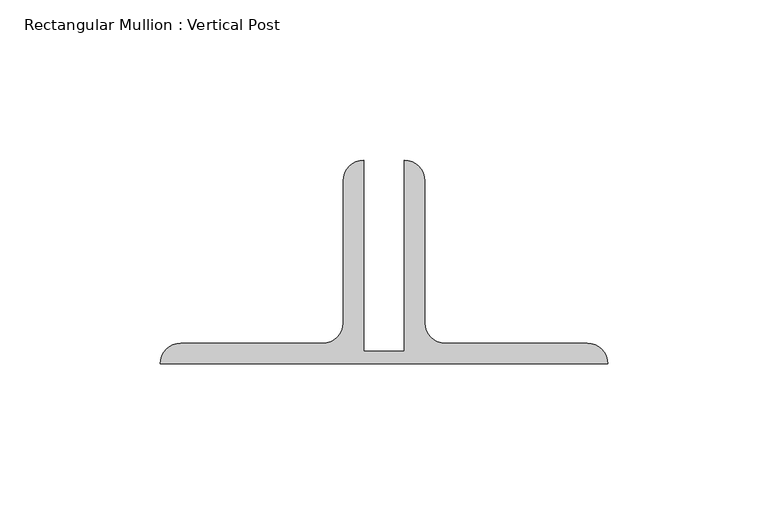
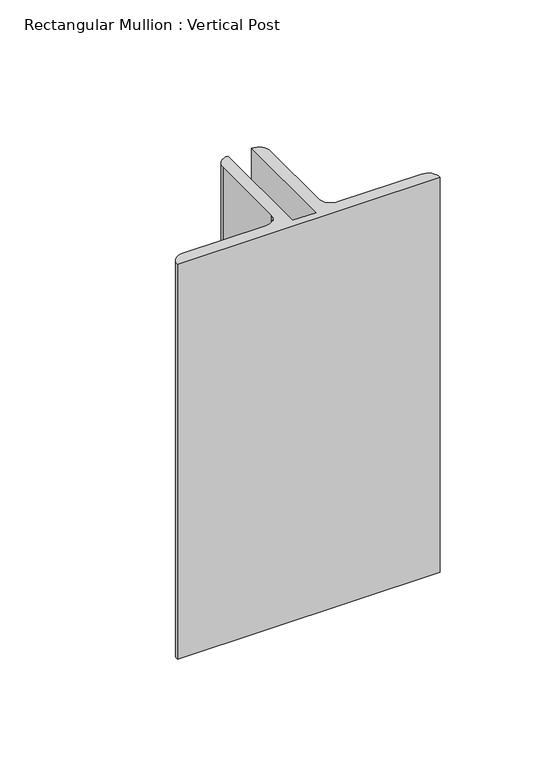
"""IFC4 building model written with IfcOpenShell, lengths in millimetres: member geometry, Rectangular Mullion : Vertical Post."""

from ifc_helpers import new_model, si_unit, point, frame, frame_2d, origin, place, context, project, spatial, polyline, circle_curve, trimmed, segment, composite_curve, outline, extrude, source, transform, mapped, element, save


def rectangular_mullion_vertical_post_21cc10da(model_context):
    return source(origin(), model_context, "Body", "SweptSolid", [
        extrude(outline(composite_curve([segment(polyline([(-76.2, 22.9145205), (-63.5, 22.9145205), (-63.5, 82.55)]), True, "CONTINUOUS"), segment(trimmed(circle_curve(frame_2d((-63.5, 76.2)), 6.35), [point((-63.5, 82.55))], [point((-57.15, 76.2))], False, "CARTESIAN"), True, "CONTINUOUS"), segment(polyline([(-57.15, 76.2), (-57.15, 31.75)]), True, "CONTINUOUS"), segment(trimmed(circle_curve(frame_2d((-50.8, 31.75)), 6.35), [point((-57.15, 31.75))], [point((-50.8, 25.4))], True, "CARTESIAN"), True, "CONTINUOUS"), segment(polyline([(-50.8, 25.4), (-6.35, 25.4)]), True, "CONTINUOUS"), segment(trimmed(circle_curve(frame_2d((-6.35, 19.05)), 6.35), [point((-6.35, 25.4))], [point((0.0, 19.05))], False, "CARTESIAN"), True, "CONTINUOUS"), segment(polyline([(0.0, 19.05), (-139.7, 19.05)]), True, "CONTINUOUS"), segment(trimmed(circle_curve(frame_2d((-133.35, 19.05)), 6.35), [point((-139.7, 19.05))], [point((-133.35, 25.4))], False, "CARTESIAN"), True, "CONTINUOUS"), segment(polyline([(-133.35, 25.4), (-88.9, 25.4)]), True, "CONTINUOUS"), segment(trimmed(circle_curve(frame_2d((-88.9, 31.75)), 6.35), [point((-88.9, 25.4))], [point((-82.55, 31.75))], True, "CARTESIAN"), True, "CONTINUOUS"), segment(polyline([(-82.55, 31.75), (-82.55, 76.2)]), True, "CONTINUOUS"), segment(trimmed(circle_curve(frame_2d((-76.2, 76.2)), 6.35), [point((-82.55, 76.2))], [point((-76.2, 82.55))], False, "CARTESIAN"), True, "CONTINUOUS"), segment(polyline([(-76.2, 82.55), (-76.2, 22.9145205)]), True, "CONTINUOUS")], self_intersect=False)), frame((0.0, 0.0, -222.0889998), z_axis=(0.0, 0.0, 1.0), x_axis=(1.0, 0.0, 0.0)), (0.0, 0.0, 1.0), 222.0889998),
    ])


if __name__ == "__main__":
    model = new_model("IFC4")
    model_context = context("Model", 3, world=origin())
    ifc_project = project(units=[si_unit("LENGTHUNIT", "METRE", prefix="MILLI")], contexts=[model_context])
    site = spatial("IfcSite", under=ifc_project)
    building = spatial("IfcBuilding", under=site)
    placement = place(None, origin())
    rectangular_mullion_vertical_post_shape = rectangular_mullion_vertical_post_21cc10da(model_context)
    element("IfcMember", 1, ObjectType="Rectangular Mullion : Vertical Post", at=placement, inside=building, context=model_context, shape_type="MappedRepresentation", body=[
        mapped(rectangular_mullion_vertical_post_shape, transform((0.0, 0.0, 0.0), x_axis=(1.0, 0.0, 0.0), y_axis=(0.0, 1.0, 0.0), z_axis=(0.0, 0.0, 1.0))),
    ])
    save(model, "model.ifc")

# Revit data of these elements
# Type "Rectangular Mullion : Vertical Post"
#   built-in parameter 1007351 = -0.0625 (stored number, unit not read)
#   built-in parameter 1007322 = 0.0126789 (stored number, unit not read)
#   built-in parameter 1007321 = 0.229167 (stored number, unit not read)
#   built-in parameter 1007320 = 0.229167 (stored number, unit not read)
# Element 1 (IfcMember, "Rectangular Mullion : Vertical Post")
#   Materials on its faces: "GATE POST: GALVANIZED ANGLES"
# Materials
#   "GATE POST: GALVANIZED ANGLES": class "Unassigned", colour RGB 211 211 211, transparency 0, Cost = 0
